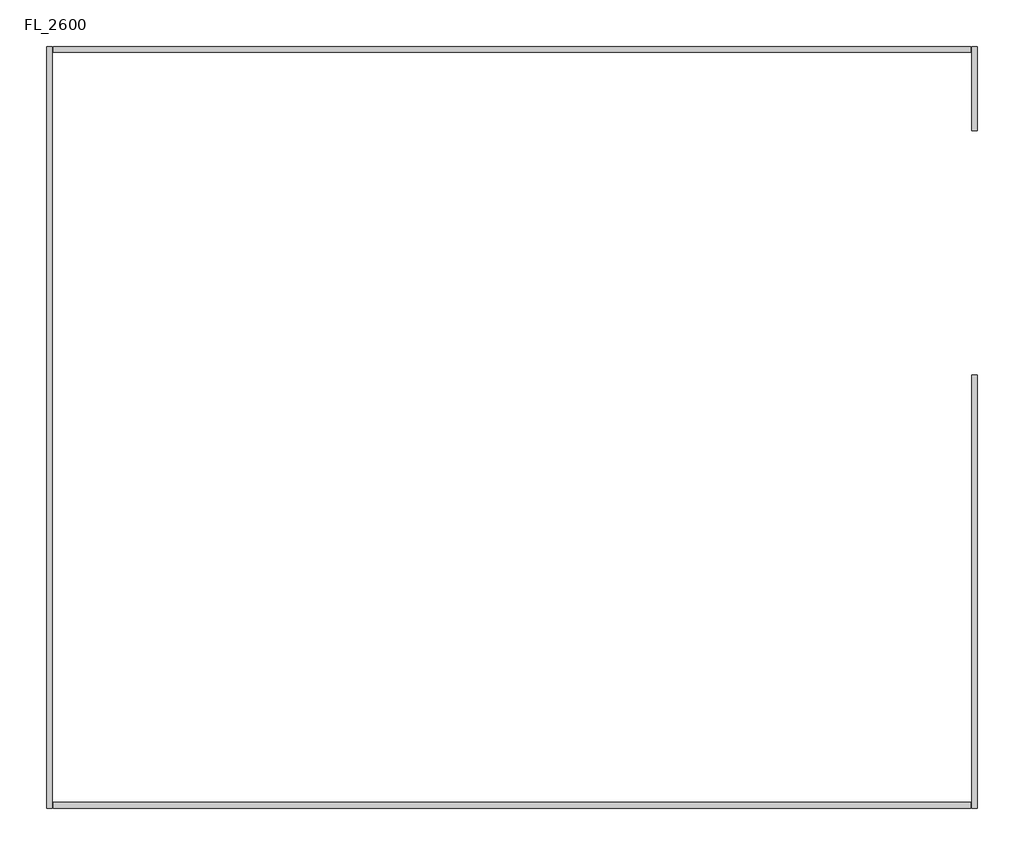
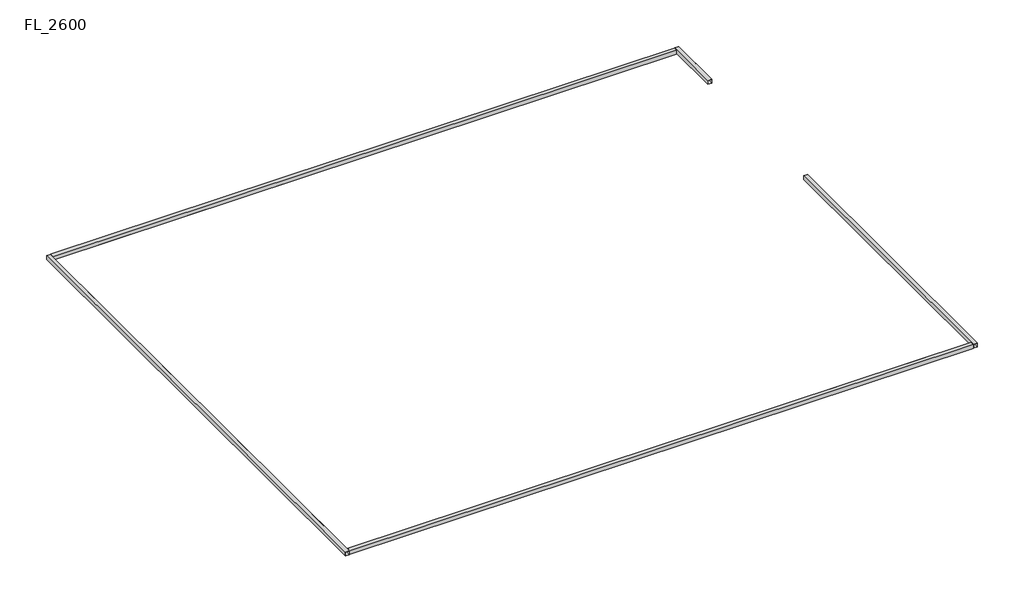
# One storey: 5 beams.
"""IFC4 building model written with IfcOpenShell, lengths in millimetres."""

import ifcopenshell
import ifcopenshell.guid

model = None  # the IFC model being written
_history = None  # IfcOwnerHistory: only IFC2X3 demands one
_inside = {}  # id of a spatial element -> (the spatial element, [elements in it])
_under = {}  # id of a project, library or spatial element -> (it, [spatial elements below it])
_declared = {}  # id of a project -> (the project, [libraries it declares])
_typed = {}  # id of a type object -> (the type object, [elements of that type])
_made_of = {}  # id of a material, layer set ... -> (it, [elements and type objects made of it])


def new_model(schema):
    """Start an empty IFC model of exactly this schema.

    Asked for "IFC4X3", IfcOpenShell would pick the latest addendum, in which some entities
    have other attributes; the version numbers below select the first issue.
    IFC2X3 requires an IfcOwnerHistory on every rooted entity: one is made here for all.
    """
    global model, _history
    if schema == "IFC4X3":
        model = ifcopenshell.file(schema_version=(4, 3, 0, 0))
    else:
        model = ifcopenshell.file(schema=schema)
    _inside.clear()
    _under.clear()
    _declared.clear()
    _typed.clear()
    _made_of.clear()
    _history = None
    if model.schema == "IFC2X3":
        org = make("IfcOrganization", Name="unknown")
        user = make(
            "IfcPersonAndOrganization",
            ThePerson=make("IfcPerson", FamilyName="unknown"),
            TheOrganization=org,
        )
        app = make(
            "IfcApplication",
            ApplicationDeveloper=org,
            Version="unknown",
            ApplicationFullName="unknown",
            ApplicationIdentifier="unknown",
        )
        _history = make(
            "IfcOwnerHistory",
            OwningUser=user,
            OwningApplication=app,
            ChangeAction="ADDED",
            CreationDate=0,
        )
    return model


def make(cls, **values):
    """One entity of the class cls with the attributes given. An attribute that is None is left unset."""
    return model.create_entity(
        cls, **{name: value for name, value in values.items() if value is not None}
    )


def rooted(cls, **values):
    """An entity with a GlobalId (a new one), such as an element, a storey or a relation."""
    return make(cls, GlobalId=ifcopenshell.guid.new(), OwnerHistory=_history, **values)


def si_unit(unit_type, name, prefix=None):
    """IfcSIUnit, for example si_unit("LENGTHUNIT", "METRE", prefix="MILLI")."""
    return make("IfcSIUnit", UnitType=unit_type, Prefix=prefix, Name=name)


def assignment(units):
    """IfcUnitAssignment: the units of a project."""
    return None if units is None else make("IfcUnitAssignment", Units=units)


def point(xyz):
    """IfcCartesianPoint."""
    return None if xyz is None else make("IfcCartesianPoint", Coordinates=xyz)


def direction(xyz):
    """IfcDirection."""
    return None if xyz is None else make("IfcDirection", DirectionRatios=xyz)


def frame(location, z_axis=None, x_axis=None):
    """IfcAxis2Placement3D, a coordinate frame: its origin and axes. An axis left out is left unset."""
    return make(
        "IfcAxis2Placement3D",
        Location=point(location),
        Axis=direction(z_axis),
        RefDirection=direction(x_axis),
    )


def origin():
    """The frame at (0, 0, 0) with its axes left unset."""
    return frame((0.0, 0.0, 0.0))


def place(relative_to, where):
    """IfcLocalPlacement: puts the frame where relative to a parent placement (None: the world)."""
    return make(
        "IfcLocalPlacement", PlacementRelTo=relative_to, RelativePlacement=where
    )


def context(
    kind, dimensions, precision=None, world=None, true_north=None, identifier=None
):
    """IfcGeometricRepresentationContext, for example the 3D "Model" context."""
    return make(
        "IfcGeometricRepresentationContext",
        ContextIdentifier=identifier,
        ContextType=kind,
        CoordinateSpaceDimension=dimensions,
        Precision=precision,
        WorldCoordinateSystem=world,
        TrueNorth=true_north,
    )


def project(units=None, contexts=None):
    """IfcProject with its units and contexts."""
    return rooted(
        "IfcProject",
        Name="project",
        RepresentationContexts=contexts,
        UnitsInContext=assignment(units),
    )


def spatial(cls, under=None, at=None, **own):
    """A site, building, storey or space (cls), placed at a placement, below another one or the project."""
    s = rooted(cls, ObjectPlacement=at, **own)
    if under is not None:
        _under.setdefault(under.id(), (under, []))[1].append(s)
    return s


def polyline(points):
    """IfcPolyline through the points."""
    return make("IfcPolyline", Points=[point(p) for p in points])


def outline(outer, holes=None, kind="AREA"):
    """IfcArbitraryClosedProfileDef: a profile drawn as a closed curve; with holes, ...WithVoids."""
    if holes is None:
        return make("IfcArbitraryClosedProfileDef", ProfileType=kind, OuterCurve=outer)
    return make(
        "IfcArbitraryProfileDefWithVoids",
        ProfileType=kind,
        OuterCurve=outer,
        InnerCurves=holes,
    )


def extrude(swept, where, along, depth):
    """IfcExtrudedAreaSolid: the profile swept, set in the frame where, extruded along a direction by depth."""
    return make(
        "IfcExtrudedAreaSolid",
        SweptArea=swept,
        Position=where,
        ExtrudedDirection=direction(along),
        Depth=depth,
    )


def shape(context_of_items, identifier, shape_type, items):
    """IfcShapeRepresentation: the items that make up one representation, for example the "Body"."""
    return make(
        "IfcShapeRepresentation",
        ContextOfItems=context_of_items,
        RepresentationIdentifier=identifier,
        RepresentationType=shape_type,
        Items=items,
    )


def source(mapping_origin, context_of_items, identifier, shape_type, items):
    """IfcRepresentationMap: a shape defined once, which mapped items show again and again."""
    return make(
        "IfcRepresentationMap",
        MappingOrigin=mapping_origin,
        MappedRepresentation=shape(context_of_items, identifier, shape_type, items),
    )


def transform(
    local_origin,
    x_axis=None,
    y_axis=None,
    z_axis=None,
    scale=None,
    scale2=None,
    scale3=None,
    uniform=True,
):
    """IfcCartesianTransformationOperator3D, or its non-uniform kind. x_axis, y_axis, z_axis: its Axis1, 2, 3."""
    if uniform:
        return make(
            "IfcCartesianTransformationOperator3D",
            Axis1=direction(x_axis),
            Axis2=direction(y_axis),
            LocalOrigin=point(local_origin),
            Scale=scale,
            Axis3=direction(z_axis),
        )
    return make(
        "IfcCartesianTransformationOperator3DnonUniform",
        Axis1=direction(x_axis),
        Axis2=direction(y_axis),
        LocalOrigin=point(local_origin),
        Scale=scale,
        Axis3=direction(z_axis),
        Scale2=scale2,
        Scale3=scale3,
    )


def mapped(mapping_source, mapping_target):
    """IfcMappedItem: shows the shape of a source again, moved by a transform."""
    return make(
        "IfcMappedItem", MappingSource=mapping_source, MappingTarget=mapping_target
    )


def made_of(thing, what):
    """Note that an element or type object is made of a material, layer set ...; save() writes the relation."""
    if what is not None:
        _made_of.setdefault(what.id(), (what, []))[1].append(thing)
    return thing


def element(
    cls,
    number,
    at=None,
    inside=None,
    cuts=None,
    type_object=None,
    material=None,
    context=None,
    identifier="Body",
    shape_type=None,
    held_by="IfcProductDefinitionShape",
    body=None,
    shapes=None,
    **own,
):
    """One element of the class cls, such as IfcWall. Its Tag is "e" and its number.

    at: its placement. inside: the storey or other place that contains it. cuts: it is an
    opening in that element (IfcRelVoidsElement). A single representation is given by context,
    identifier, shape_type and body (its items); several are given by shapes. held_by: the class
    of the entity that holds the representations. save() writes the other relations.
    """
    e = rooted(cls, Tag="e%d" % number, ObjectPlacement=at, **own)
    if body is not None:
        shapes = [shape(context, identifier, shape_type, body)]
    if shapes is not None:
        e.Representation = make(held_by, Representations=shapes)
    if inside is not None:
        _inside.setdefault(inside.id(), (inside, []))[1].append(e)
    if cuts is not None:
        rooted(
            "IfcRelVoidsElement", RelatingBuildingElement=cuts, RelatedOpeningElement=e
        )
    if type_object is not None:
        _typed.setdefault(type_object.id(), (type_object, []))[1].append(e)
    return made_of(e, material)


def aggregate(whole, parts):
    """IfcRelAggregates: a whole, such as a stair, and the parts it consists of."""
    return rooted("IfcRelAggregates", RelatingObject=whole, RelatedObjects=parts)


def save(model, path):
    """Write the relations noted so far, then the file.

    IfcRelAggregates (storeys below a building ...), IfcRelContainedInSpatialStructure (elements
    in a storey), IfcRelDefinesByType, IfcRelAssociatesMaterial and IfcRelDeclares: one each for
    every whole, place, type object, material and project.
    """
    for whole, parts in _under.values():
        aggregate(whole, parts)
    for where, things in _inside.values():
        rooted(
            "IfcRelContainedInSpatialStructure",
            RelatedElements=things,
            RelatingStructure=where,
        )
    for kind, things in _typed.values():
        rooted("IfcRelDefinesByType", RelatedObjects=things, RelatingType=kind)
    for what, things in _made_of.values():
        rooted("IfcRelAssociatesMaterial", RelatedObjects=things, RelatingMaterial=what)
    for by, libraries in _declared.values():
        rooted("IfcRelDeclares", RelatingContext=by, RelatedDefinitions=libraries)
    model.write(path)


def steel_rectangular_beam_bm125_rt_100x100x4_0_fd47acba(model_context):
    return source(origin(), model_context, "Body", "SweptSolid", [
        extrude(outline(polyline([(-50.0, 50.0), (50.0, 50.0), (50.0, -50.0), (-50.0, -50.0), (-50.0, 50.0)]), holes=[polyline([(46.0, -46.0), (46.0, 46.0), (-46.0, 46.0), (-46.0, -46.0), (46.0, -46.0)])]), frame((-7887.3, 0.0, 0.0), z_axis=(1.0, 0.0, 0.0), x_axis=(0.0, 1.0, 0.0)), (0.0, 0.0, 1.0), 15774.6),
        extrude(outline(polyline([(-50.0, 50.0), (50.0, 50.0), (50.0, -50.0), (-50.0, -50.0), (-50.0, 50.0)]), holes=[polyline([(46.0, -46.0), (46.0, 46.0), (-46.0, 46.0), (-46.0, -46.0), (46.0, -46.0)])]), frame((-7887.3, 0.0, 0.0), z_axis=(1.0, 0.0, 0.0), x_axis=(0.0, 1.0, 0.0)), (0.0, 0.0, 1.0), 15774.6),
        extrude(outline(polyline([(-50.0, 50.0), (50.0, 50.0), (50.0, -50.0), (-50.0, -50.0), (-50.0, 50.0)]), holes=[polyline([(46.0, -46.0), (46.0, 46.0), (-46.0, 46.0), (-46.0, -46.0), (46.0, -46.0)])]), frame((-7887.3, 0.0, 0.0), z_axis=(1.0, 0.0, 0.0), x_axis=(0.0, 1.0, 0.0)), (0.0, 0.0, 1.0), 15774.6),
        extrude(outline(polyline([(-50.0, 50.0), (50.0, 50.0), (50.0, -50.0), (-50.0, -50.0), (-50.0, 50.0)]), holes=[polyline([(46.0, -46.0), (46.0, 46.0), (-46.0, 46.0), (-46.0, -46.0), (46.0, -46.0)])]), frame((-7887.3, 0.0, 0.0), z_axis=(1.0, 0.0, 0.0), x_axis=(0.0, 1.0, 0.0)), (0.0, 0.0, 1.0), 15774.6),
    ])


def steel_rectangular_beam_bm125_rt_100x100x4_0_2c93a6f0(model_context):
    return source(origin(), model_context, "Body", "SweptSolid", [
        extrude(outline(polyline([(-50.0, 50.0), (50.0, 50.0), (50.0, -50.0), (-50.0, -50.0), (-50.0, 50.0)]), holes=[polyline([(46.0, -46.0), (46.0, 46.0), (-46.0, 46.0), (-46.0, -46.0), (46.0, -46.0)])]), frame((-6550.0, 0.0, 0.0), z_axis=(1.0, 0.0, 0.0), x_axis=(0.0, 1.0, 0.0)), (0.0, 0.0, 1.0), 13100.0),
        extrude(outline(polyline([(-50.0, 50.0), (50.0, 50.0), (50.0, -50.0), (-50.0, -50.0), (-50.0, 50.0)]), holes=[polyline([(46.0, -46.0), (46.0, 46.0), (-46.0, 46.0), (-46.0, -46.0), (46.0, -46.0)])]), frame((-6550.0, 0.0, 0.0), z_axis=(1.0, 0.0, 0.0), x_axis=(0.0, 1.0, 0.0)), (0.0, 0.0, 1.0), 13100.0),
        extrude(outline(polyline([(-50.0, 50.0), (50.0, 50.0), (50.0, -50.0), (-50.0, -50.0), (-50.0, 50.0)]), holes=[polyline([(46.0, -46.0), (46.0, 46.0), (-46.0, 46.0), (-46.0, -46.0), (46.0, -46.0)])]), frame((-6550.0, 0.0, 0.0), z_axis=(1.0, 0.0, 0.0), x_axis=(0.0, 1.0, 0.0)), (0.0, 0.0, 1.0), 13100.0),
        extrude(outline(polyline([(-50.0, 50.0), (50.0, 50.0), (50.0, -50.0), (-50.0, -50.0), (-50.0, 50.0)]), holes=[polyline([(46.0, -46.0), (46.0, 46.0), (-46.0, 46.0), (-46.0, -46.0), (46.0, -46.0)])]), frame((-6550.0, 0.0, 0.0), z_axis=(1.0, 0.0, 0.0), x_axis=(0.0, 1.0, 0.0)), (0.0, 0.0, 1.0), 13100.0),
    ])


def steel_rectangular_beam_bm125_rt_100x100x4_0_60a5dd41(model_context):
    return source(origin(), model_context, "Body", "SweptSolid", [
        extrude(outline(polyline([(-50.0, 50.0), (50.0, 50.0), (50.0, -50.0), (-50.0, -50.0), (-50.0, 50.0)]), holes=[polyline([(46.0, -46.0), (46.0, 46.0), (-46.0, 46.0), (-46.0, -46.0), (46.0, -46.0)])]), frame((-3725.0, 0.0, 0.0), z_axis=(1.0, 0.0, 0.0), x_axis=(0.0, 1.0, 0.0)), (0.0, 0.0, 1.0), 7450.0),
        extrude(outline(polyline([(-50.0, 50.0), (50.0, 50.0), (50.0, -50.0), (-50.0, -50.0), (-50.0, 50.0)]), holes=[polyline([(46.0, -46.0), (46.0, 46.0), (-46.0, 46.0), (-46.0, -46.0), (46.0, -46.0)])]), frame((-3725.0, 0.0, 0.0), z_axis=(1.0, 0.0, 0.0), x_axis=(0.0, 1.0, 0.0)), (0.0, 0.0, 1.0), 7450.0),
        extrude(outline(polyline([(-50.0, 50.0), (50.0, 50.0), (50.0, -50.0), (-50.0, -50.0), (-50.0, 50.0)]), holes=[polyline([(46.0, -46.0), (46.0, 46.0), (-46.0, 46.0), (-46.0, -46.0), (46.0, -46.0)])]), frame((-3725.0, 0.0, 0.0), z_axis=(1.0, 0.0, 0.0), x_axis=(0.0, 1.0, 0.0)), (0.0, 0.0, 1.0), 7450.0),
        extrude(outline(polyline([(-50.0, 50.0), (50.0, 50.0), (50.0, -50.0), (-50.0, -50.0), (-50.0, 50.0)]), holes=[polyline([(46.0, -46.0), (46.0, 46.0), (-46.0, 46.0), (-46.0, -46.0), (46.0, -46.0)])]), frame((-3725.0, 0.0, 0.0), z_axis=(1.0, 0.0, 0.0), x_axis=(0.0, 1.0, 0.0)), (0.0, 0.0, 1.0), 7450.0),
    ])


def steel_rectangular_beam_bm125_rt_100x100x4_0_366960fc(model_context):
    return source(origin(), model_context, "Body", "SweptSolid", [
        extrude(outline(polyline([(-50.0, 50.0), (50.0, 50.0), (50.0, -50.0), (-50.0, -50.0), (-50.0, 50.0)]), holes=[polyline([(46.0, -46.0), (46.0, 46.0), (-46.0, 46.0), (-46.0, -46.0), (46.0, -46.0)])]), frame((-725.0, 0.0, 0.0), z_axis=(1.0, 0.0, 0.0), x_axis=(0.0, 1.0, 0.0)), (0.0, 0.0, 1.0), 1450.0),
        extrude(outline(polyline([(-50.0, 50.0), (50.0, 50.0), (50.0, -50.0), (-50.0, -50.0), (-50.0, 50.0)]), holes=[polyline([(46.0, -46.0), (46.0, 46.0), (-46.0, 46.0), (-46.0, -46.0), (46.0, -46.0)])]), frame((-725.0, 0.0, 0.0), z_axis=(1.0, 0.0, 0.0), x_axis=(0.0, 1.0, 0.0)), (0.0, 0.0, 1.0), 1450.0),
        extrude(outline(polyline([(-50.0, 50.0), (50.0, 50.0), (50.0, -50.0), (-50.0, -50.0), (-50.0, 50.0)]), holes=[polyline([(46.0, -46.0), (46.0, 46.0), (-46.0, 46.0), (-46.0, -46.0), (46.0, -46.0)])]), frame((-725.0, 0.0, 0.0), z_axis=(1.0, 0.0, 0.0), x_axis=(0.0, 1.0, 0.0)), (0.0, 0.0, 1.0), 1450.0),
        extrude(outline(polyline([(-50.0, 50.0), (50.0, 50.0), (50.0, -50.0), (-50.0, -50.0), (-50.0, 50.0)]), holes=[polyline([(46.0, -46.0), (46.0, 46.0), (-46.0, 46.0), (-46.0, -46.0), (46.0, -46.0)])]), frame((-725.0, 0.0, 0.0), z_axis=(1.0, 0.0, 0.0), x_axis=(0.0, 1.0, 0.0)), (0.0, 0.0, 1.0), 1450.0),
    ])


model = new_model("IFC4")

# Units and contexts
model_context = context("Model", 3, world=origin())
ifc_project = project(units=[si_unit("LENGTHUNIT", "METRE", prefix="MILLI")], contexts=[model_context])

# Site, building, storey
site = spatial("IfcSite", under=ifc_project)
building = spatial("IfcBuilding", under=site)
storey = spatial("IfcBuildingStorey", under=building, Name="FL_2600", Elevation=2600.0)

# Beams
placement = place(None, origin())
steel_rectangular_beam_bm125_rt_100x100x4_0_shape = steel_rectangular_beam_bm125_rt_100x100x4_0_fd47acba(model_context)
element("IfcBeam", 1, ObjectType="Steel-Rectangular-Beam : BM125_RT-100x100x4.0", at=placement, inside=storey, context=model_context, shape_type="MappedRepresentation", body=[
    mapped(steel_rectangular_beam_bm125_rt_100x100x4_0_shape, transform((6100.0, 10094.5382614, 2550.0), x_axis=(1.0, 0.0, 0.0), y_axis=(0.0, 1.0, 0.0), z_axis=(0.0, 0.0, 1.0))),
])
element("IfcBeam", 2, ObjectType="Steel-Rectangular-Beam : BM125_RT-100x100x4.0", at=placement, inside=storey, context=model_context, shape_type="MappedRepresentation", body=[
    mapped(steel_rectangular_beam_bm125_rt_100x100x4_0_shape, transform((6100.0, 23094.5382614, 2550.0), x_axis=(-1.0, 0.0, 0.0), y_axis=(0.0, -1.0, 0.0), z_axis=(0.0, 0.0, 1.0))),
])
steel_rectangular_beam_bm125_rt_100x100x4_0_2_shape = steel_rectangular_beam_bm125_rt_100x100x4_0_2c93a6f0(model_context)
element("IfcBeam", 3, ObjectType="Steel-Rectangular-Beam : BM125_RT-100x100x4.0", at=placement, inside=storey, context=model_context, shape_type="MappedRepresentation", body=[
    mapped(steel_rectangular_beam_bm125_rt_100x100x4_0_2_shape, transform((-1850.0, 16594.5382614, 2550.0), x_axis=(0.0, -1.0, 0.0), y_axis=(1.0, 0.0, 0.0), z_axis=(0.0, 0.0, 1.0))),
])
steel_rectangular_beam_bm125_rt_100x100x4_0_3_shape = steel_rectangular_beam_bm125_rt_100x100x4_0_60a5dd41(model_context)
element("IfcBeam", 4, ObjectType="Steel-Rectangular-Beam : BM125_RT-100x100x4.0", at=placement, inside=storey, context=model_context, shape_type="MappedRepresentation", body=[
    mapped(steel_rectangular_beam_bm125_rt_100x100x4_0_3_shape, transform((14050.0, 13769.5382614, 2550.0), x_axis=(0.0, 1.0, 0.0), y_axis=(-1.0, 0.0, 0.0), z_axis=(0.0, 0.0, 1.0))),
])
steel_rectangular_beam_bm125_rt_100x100x4_0_4_shape = steel_rectangular_beam_bm125_rt_100x100x4_0_366960fc(model_context)
element("IfcBeam", 5, ObjectType="Steel-Rectangular-Beam : BM125_RT-100x100x4.0", at=placement, inside=storey, context=model_context, shape_type="MappedRepresentation", body=[
    mapped(steel_rectangular_beam_bm125_rt_100x100x4_0_4_shape, transform((14050.0, 22419.5382614, 2550.0), x_axis=(0.0, 1.0, 0.0), y_axis=(-1.0, 0.0, 0.0), z_axis=(0.0, 0.0, 1.0))),
])

save(model, "model.ifc")

# Revit data of these elements
# Project information
#   Project ISM Data = "<?xml version=\"1.0\" encoding=\"utf-16\"?><ism schema_version=\"03.00\"><section_positioning><element family_name=\"CO_RC_REC\" symbol_name=\"CCC12_Rec_450x450\" section_id=\"F2ADF140-E21A-4820-8170-6F63D956DCAD\" category=\"OST_StructuralColumns\" mirror_y=\"0\" mirror_x=\"0\" /><element family_name=\"CO_RC_REC\" symbol_name=\"CCC12_Rec_450x450\" section_id=\"B35A310E-4F33-462b-819C-3ADD300C0CEB\" category=\"OST_StructuralColumns\" mirror_y=\"0\" mirror_x=\"0\" /><element family_name=\"CO_RC_REC\" symbol_name=\"CCC12_Rec_450x450\" section_id=\"711054EC-0DB2-46e3-AD20-004560300C00\" category=\"OST_StructuralColumns\" mirror_y=\"0\" mirror_x=\"0\" /><element family_name=\"CO_RC_REC\" symbol_name=\"300 x 450\" section_id=\"B5C54EC9-8EBD-4860-AB72-EF5791AED394\" category=\"OST_StructuralColumns\" mirror_y=\"0\" mirror_x=\"0\" /><element family_name=\"GI_RC_C\" symbol_name=\"SGC11_400x500\" section_id=\"0A7B8D02-9EA4-4aa9-A41A-E30BB5B6B6C5\" category=\"OST_StructuralFraming\" mirror_y=\"0\" mirror_x=\"0\" /><element family_name=\"GI_RC_C\" symbol_name=\"SGC11_400x500\" section_id=\"714BBD27-DB58-47da-B54C-5806291C2D3C\" category=\"OST_StructuralFraming\" mirror_y=\"0\" mirror_x=\"0\" /><element family_name=\"GI_RC_C\" symbol_name=\"SGC11_400x500\" section_id=\"F36E62C1-13EE-4807-A3C1-899E23E0BEDE\" category=\"OST_StructuralFraming\" mirror_y=\"0\" mirror_x=\"0\" /><element family_name=\"GI_RC_C\" symbol_name=\"SGC11_400x500\" section_id=\"F5448801-679E-44d6-8F46-E676344F8165\" category=\"OST_StructuralFraming\" mirror_y=\"0\" mirror_x=\"0\" /><element family_name=\"GI_RC_C\" symbol_name=\"SGC11_400x600\" section_id=\"05D74241-6318-4cac-95F5-7B878260D5B5\" category=\"OST_StructuralFraming\" mirror_y=\"0\" mirror_x=\"0\" /><element family_name=\"GI_RC_C\" symbol_name=\"SGC11_400x500\" section_id=\"846DCB0C-E06B-4978-9D43-E1CC0FDE7595\" category=\"OST_StructuralFraming\" mirror_y=\"0\" mirror_x=\"0\" /><element family_name=\"GI_RC_C\" symbol_name=\"SGC11_400x500\" section_id=\"2ADF82B8-986D-4f44-85DE-89D921292160\" category=\"OST_StructuralFraming\" mirror_y=\"0\" mirror_x=\"0\" /><element family_name=\"GI_RC_C\" symbol_name=\"SGC11_400x500\" section_id=\"7AF371ED-051B-4a30-8826-11F11C212B73\" category=\"OST_StructuralFraming\" mirror_y=\"0\" mirror_x=\"0\" /><element family_name=\"GI_RC_C\" symbol_name=\"SGC11_400x500\" section_id=\"2FE74006-ADDA-412f-A522-853919E62B4D\" category=\"OST_StructuralFraming\" mirror_y=\"0\" mirror_x=\"0\" /><element family_name=\"GI_RC_C\" symbol_name=\"SGC11_400x500\" section_id=\"09B63641-D581-4a6c-A18E-54C17EC989A4\" category=\"OST_StructuralFraming\" mirror_y=\"0\" mirror_x=\"0\" /><element family_name=\"GI_RC_C\" symbol_name=\"SGC11_400x500\" section_id=\"0DD6B52A-77D0-45a1-82B1-8236ED57078C\" category=\"OST_StructuralFraming\" mirror_y=\"0\" mirror_x=\"0\" /><element family_name=\"GI_RC_C\" symbol_name=\"SGC11_400x500\" section_id=\"35D311D2-DEB8-4469-97DE-110B6DF5B84D\" category=\"OST_StructuralFraming\" mirror_y=\"0\" mirror_x=\"0\" /><element family_name=\"GI_RC_C\" symbol_name=\"SGC11_400x500\" section_id=\"0D3CCDE5-CFF9-431b-A4BD-01BF6636D6BD\" category=\"OST_StructuralFraming\" mirror_y=\"0\" mirror_x=\"0\" /><element family_name=\"GI_RC_C\" symbol_name=\"SGC11_400x500\" section_id=\"C62B2A5B-024A-47ac-B030-C17A67E64A7B\" category=\"OST_StructuralFraming\" mirror_y=\"0\" mirror_x=\"0\" /><element family_name=\"GI_RC_C\" symbol_name=\"SGC11_400x500\" section_id=\"944C6E43-E607-48c3-8358-9E6CB88346E7\" category=\"OST_StructuralFraming\" mirror_y=\"0\" mirror_x=\"0\" /><element family_name=\"GI_RC_C\" symbol_name=\"SGC11_400x500\" section_id=\"A4B1F42D-B1C2-4ad2-8AD6-DB0D5E05998D\" category=\"OST_StructuralFraming\" mirror_y=\"0\" mirror_x=\"0\" /><element family_name=\"GI_RC_C\" symbol_name=\"SGC11_400x500\" section_id=\"007E6C70-1139-4b48-B003-C76FAD4C249A\" category=\"OST_StructuralFraming\" mirror_y=\"0\" mirror_x=\"0\" /><element family_name=\"GI_RC_C\" symbol_name=\"SGC11_400x500\" section_id=\"9941AC94-F03A-464c-9912-04590E0C31E0\" category=\"OST_StructuralFraming\" mirror_y=\"0\" mirror_x=\"0\" /><element family_name=\"GI_RC_C\" symbol_name=\"SGC11_400x500\" section_id=\"CFD98B8D-8FF4-4e71-A909-0FE7DBCE924E\" category=\"OST_StructuralFraming\" mirror_y=\"0\" mirror_x=\"0\" /><element family_name=\"GI_RC_C\" symbol_name=\"SGC11_400x500\" section_id=\"58262161-98E6-45c8-B2BD-4508105FF662\" category=\"OST_StructuralFraming\" mirror_y=\"0\" mirror_x=\"0\" /><element family_name=\"GI_RC_C\" symbol_name=\"SGC11_400x500\" section_id=\"66AB4841-610A-4883-97F7-1282A56484E1\" category=\"OST_StructuralFraming\" mirror_y=\"0\" mirror_x=\"0\" /><element family_name=\"GI_RC_C\" symbol_name=\"SGC11_400x500\" section_id=\"D2B324BE-BBD6-49da-9730-60EA7AD4D3A0\" category=\"OST_StructuralFraming\" mirror_y=\"0\" mirror_x=\"0\" /><element family_name=\"GI_RC_C\" symbol_name=\"SGC11_400x500\" section_id=\"92A8ECE7-C053-46b1-92ED-F2C041617E7B\" category=\"OST_StructuralFraming\" mirror_y=\"0\" mirror_x=\"0\" /><element family_name=\"GI_RC_C\" symbol_name=\"SGC11_400x500\" section_id=\"B4C4BDB0-65C4-4016-9C78-DBD77E229523\" category=\"OST_StructuralFraming\" mirror_y=\"0\" mirror_x=\"0\" /><element family_name=\"GI_RC_C\" symbol_name=\"SGC11_400x500\" section_id=\"57270646-162F-4c83-BDB7-A5FBEA9120BD\" category=\"OST_StructuralFraming\" mirror_y=\"0\" mirror_x=\"0\" /><element family_name=\"GI_RC_C\" symbol_name=\"SGC11_400x500\" section_id=\"BDEF733F-00AA-4eee-B6C6-50229FC1D236\" category=\"OST_StructuralFraming\" mirror_y=\"0\" mirror_x=\"0\" /><element family_name=\"GI_RC_C\" symbol_name=\"SGC11_400x500\" section_id=\"84A94E1E-3074-40f4-9690-97191755F019\" category=\"OST_StructuralFraming\" mirror_y=\"0\" mirror_x=\"0\" /><element family_name=\"GI_RC_C\" symbol_name=\"SGC11_400x500\" section_id=\"8A7D913D-7967-4718-912D-B83DF0AD2EDD\" category=\"OST_StructuralFraming\" mirror_y=\"0\" mirror_x=\"0\" /><element family_name=\"GI_RC_C\" symbol_name=\"SGC11_400x500\" section_id=\"83553D70-90FA-469c-B5C3-EF03F3FC6475\" category=\"OST_StructuralFraming\" mirror_y=\"0\" mirror_x=\"0\" /><element family_name=\"GI_RC_C\" symbol_name=\"SGC11_400x500\" section_id=\"6880C1E4-C50B-4c1b-B61C-23F2D8C46873\" category=\"OST_StructuralFraming\" mirror_y=\"0\" mirror_x=\"0\" /><element family_name=\"GI_RC_C\" symbol_name=\"SGC11_400x500\" section_id=\"08594C43-CD40-47de-A3BA-8BFB47F64994\" category=\"OST_StructuralFraming\" mirror_y=\"0\" mirror_x=\"0\" /><element family_name=\"GI_RC_C\" symbol_name=\"SGC11_400x500\" section_id=\"7D2E11FA-A5E1-4434-B9BE-AABA1A16CA03\" category=\"OST_StructuralFraming\" mirror_y=\"0\" mirror_x=\"0\" /><element family_name=\"GI_RC_C\" symbol_name=\"SGC11_400x500\" section_id=\"D892DFA4-5441-4ad2-A390-253492293B1B\" category=\"OST_StructuralFraming\" mirror_y=\"0\" mirror_x=\"0\" /><element family_name=\"GI_RC_C\" symbol_name=\"SGC11_400x500\" section_id=\"E5A32FE6-89C4-49f1-B3B9-1CABE7C48A4D\" category=\"OST_StructuralFraming\" mirror_y=\"0\" mirror_x=\"0\" /><element family_name=\"GI_RC_C\" symbol_name=\"SGC11_400x500\" section_id=\"8AE872C2-5DBE-47c5-934B-7E964A84B589\" category=\"OST_StructuralFraming\" mirror_y=\"0\" mirror_x=\"0\" /><element family_name=\"GI_RC_C\" symbol_name=\"SGC11_400x500\" section_id=\"3C847B60-488A-4604-A400-16A3A65E919B\" category=\"OST_StructuralFraming\" mirror_y=\"0\" mirror_x=\"0\" /><element family_name=\"GI_RC_C\" symbol_name=\"SGC11_400x500\" section_id=\"DBEC432A-3F7B-4266-AD99-2A937DC70BCF\" category=\"OST_StructuralFraming\" mirror_y=\"0\" mirror_x=\"0\" /><element family_name=\"GI_RC_C\" symbol_name=\"SGC11_400x500\" section_id=\"59403DD6-7A51-48aa-A3BE-962457E6F10E\" category=\"OST_StructuralFraming\" mirror_y=\"0\" mirror_x=\"0\" /><element family_name=\"GI_RC_C\" symbol_name=\"SGC11_400x500\" section_id=\"11CDDF5D-38B6-43b2-A291-FC188BE232BC\" category=\"OST_StructuralFraming\" mirror_y=\"0\" mirror_x=\"0\" /><element family_name=\"GI_RC_C\" symbol_name=\"SGC11_400x500\" section_id=\"10BF2843-EFC9-4136-933C-5B270D970277\" category=\"OST_StructuralFraming\" mirror_y=\"0\" mirror_x=\"0\" /><element family_name=\"GI_RC_C\" symbol_name=\"SGC11_400x500\" section_id=\"E1B09A9C-F6C6-47d9-976B-E313C0E3F52B\" category=\"OST_StructuralFraming\" mirror_y=\"0\" mirror_x=\"0\" /><element family_name=\"GI_RC_C\" symbol_name=\"SGC11_400x500\" section_id=\"A3A22EC3-26C8-4588-A0AB-AFAE02DF267E\" category=\"OST_StructuralFraming\" mirror_y=\"0\" mirror_x=\"0\" /><element family_name=\"GI_RC_C\" symbol_name=\"SGC11_400x500\" section_id=\"114828FC-BDC1-4343-9119-BCB5395DAA64\" category=\"OST_StructuralFraming\" mirror_y=\"0\" mirror_x=\"0\" /><element family_name=\"GI_RC_C\" symbol_name=\"SGC11_400x500\" section_id=\"797626F9-3558-4623-826F-15FB93088CB3\" category=\"OST_StructuralFraming\" mirror_y=\"0\" mirror_x=\"0\" /><element family_name=\"GI_RC_C\" symbol_name=\"SGC11_400x500\" section_id=\"4BF369CD-DF09-4346-96CB-C6C6380A2599\" category=\"OST_StructuralFraming\" mirror_y=\"0\" mirror_x=\"0\" /><element family_name=\"GI_RC_C\" symbol_name=\"SGC11_400x500\" section_id=\"722B46BA-61C4-44a1-9ECF-325B60B6688D\" category=\"OST_StructuralFraming\" mirror_y=\"0\" mirror_x=\"0\" /><element family_name=\"GI_RC_C\" symbol_name=\"SGC11_400x500\" section_id=\"C33DBE84-19C1-4379-AB6E-A41F7420F18C\" category=\"OST_StructuralFraming\" mirror_y=\"0\" mirror_x=\"0\" /><element family_name=\"GI_RC_C\" symbol_name=\"SGC11_400x500\" section_id=\"1F2D3B75-66F2-4d88-A1DD-647969477B86\" category=\"OST_StructuralFraming\" mirror_y=\"0\" mirror_x=\"0\" /><element family_name=\"GI_RC_C\" symbol_name=\"SGC11_400x500\" section_id=\"DFBF96B2-410A-4f39-80C4-D8CF78561C93\" category=\"OST_StructuralFraming\" mirror_y=\"0\" mirror_x=\"0\" /><element family_name=\"GI_RC_C\" symbol_name=\"SGC11_400x500\" section_id=\"D6793CD3-AB64-417c-9C28-8B18A0A2D336\" category=\"OST_StructuralFraming\" mirror_y=\"0\" mirror_x=\"0\" /><element family_name=\"GI_RC_C\" symbol_name=\"SGC11_400x500\" section_id=\"90884AC0-EA00-4caa-86E1-E6B886FD90ED\" category=\"OST_StructuralFraming\" mirror_y=\"0\" mirror_x=\"0\" /><element family_name=\"GI_RC_C\" symbol_name=\"SGC11_400x500\" section_id=\"64BC7B89-F7C8-4dae-A5C8-F10DF9E5F6BA\" category=\"OST_StructuralFraming\" mirror_y=\"0\" mirror_x=\"0\" /><element family_name=\"GI_RC_C\" symbol_name=\"SGC11_400x500\" section_id=\"D82E4D85-2728-40e5-9F60-1C7FB2990D78\" category=\"OST_StructuralFraming\" mirror_y=\"0\" mirror_x=\"0\" /><element family_name=\"GI_RC_C\" symbol_name=\"SGC11_400x500\" section_id=\"1E6D05B9-BF84-4669-AA27-948ADA1D511E\" category=\"OST_StructuralFraming\" mirror_y=\"0\" mirror_x=\"0\" /><element family_name=\"GI_RC_C\" symbol_name=\"SGC11_400x500\" section_id=\"73608CB2-EB94-466e-883D-814030EF49D6\" category=\"OST_StructuralFraming\" mirror_y=\"0\" mirror_x=\"0\" /><element family_name=\"GI_RC_C\" symbol_name=\"SGC11_400x500\" section_id=\"4EAF07EF-4E08-4065-9F08-BF69D4413867\" category=\"OST_StructuralFraming\" mirror_y=\"1\" mirror_x=\"1\" /></section_positioning><surface_member_mappings /><element_binding><element revit_id=\"0aa8b22b-49cd-4eb2-b994-d423f7aad482-0014435e\" ism_id=\"637A3C89-B4B9-4EE4-9E04-FF73E7A5771D\" /><element revit_id=\"af7cfdda-f71a-4a09-bb03-63e0c16d5d93-00152efa\" ism_id=\"088C1743-AFAE-4D55-B14F-2330F3A79060\" /><element revit_id=\"af7cfdda-f71a-4a09-bb03-63e0c16d5d93-00152efc\" ism_id=\"38278b30-864a-4bde-bfee-6c2d4309b281\" /><element revit_id=\"af7cfdda-f71a-4a09-bb03-63e0c16d5d93-00152eff\" ism_id=\"e2895b00-887b-4cf1-92a9-c4855f67b579\" /><element revit_id=\"af7cfdda-f71a-4a09-bb03-63e0c16d5d93-00152f02\" ism_id=\"a6b13b86-1938-47ee-8937-754844bb71d9\" /><element revit_id=\"af7cfdda-f71a-4a09-bb03-63e0c16d5d93-00152f05\" ism_id=\"b3cdb4ae-01be-49a8-8521-dfb37fcb7a09\" /><element revit_id=\"af7cfdda-f71a-4a09-bb03-63e0c16d5d93-00152f08\" ism_id=\"0a200294-2d0f-43b2-a10b-c345be42008c\" /><element revit_id=\"af7cfdda-f71a-4a09-bb03-63e0c16d5d
#     93-00152f0a\" ism_id=\"434ac00d-0b75-408a-b526-bf8655b26baf\" /><element revit_id=\"af7cfdda-f71a-4a09-bb03-63e0c16d5d93-00152f0c\" ism_id=\"5e4f7e2a-2154-47cc-93bc-24e7bd197632\" /><element revit_id=\"af7cfdda-f71a-4a09-bb03-63e0c16d5d93-00152f0e\" ism_id=\"f1998cd9-044c-4f7a-99e6-248bc5b45dba\" /><element revit_id=\"af7cfdda-f71a-4a09-bb03-63e0c16d5d93-00152f10\" ism_id=\"6ca0e144-6dd7-4824-b6a4-c3599ffcc64c\" /><element revit_id=\"af7cfdda-f71a-4a09-bb03-63e0c16d5d93-00152f12\" ism_id=\"173f1f07-ca52-4750-b7f6-1ef0180c36ba\" /><element revit_id=\"af7cfdda-f71a-4a09-bb03-63e0c16d5d93-00152f15\" ism_id=\"29a619d1-86ac-46c7-a220-2e78769b313e\" /><element revit_id=\"af7cfdda-f71a-4a09-bb03-63e0c16d5d93-00152f17\" ism_id=\"de21b25d-6b5e-4da6-89ee-8b671f1287ec\" /><element revit_id=\"af7cfdda-f71a-4a09-bb03-63e0c16d5d93-00152f19\" ism_id=\"70cdf538-eeaa-48c4-9315-181e56578638\" /><element revit_id=\"af7cfdda-f71a-4a09-bb03-63e0c16d5d93-00152f1b\" ism_id=\"49734cf8-a963-4163-b104-a25bff74fff0\" /><element revit_id=\"af7cfdda-f71a-4a09-bb03-63e0c16d5d93-00152f1d\" ism_id=\"a5a98e28-e98d-4759-bcab-d40632bfc19f\" /><element revit_id=\"af7cfdda-f71a-4a09-bb03-63e0c16d5d93-00152f1f\" ism_id=\"ab6af08f-90da-4d2f-a66a-db65621b8e94\" /><element revit_id=\"af7cfdda-f71a-4a09-bb03-63e0c16d5d93-00152f21\" ism_id=\"a65b64ab-134d-4223-82b7-5e66d90bc276\" /><element revit_id=\"af7cfdda-f71a-4a09-bb03-63e0c16d5d93-00152f23\" ism_id=\"6a1f317f-8940-4af8-9522-8e6c47c0c3a6\" /><element revit_id=\"af7cfdda-f71a-4a09-bb03-63e0c16d5d93-00152f25\" ism_id=\"880c6aab-7058-4382-9d83-6c759bdcf822\" /><element revit_id=\"af7cfdda-f71a-4a09-bb03-63e0c16d5d93-00152f27\" ism_id=\"555977b1-6494-4ee8-b235-8bae97762787\" /><element revit_id=\"af7cfdda-f71a-4a09-bb03-63e0c16d5d93-00152f29\" ism_id=\"66c9b467-8c65-4f1e-9542-95b43d793e9b\" /><element revit_id=\"af7cfdda-f71a-4a09-bb03-63e0c16d5d93-00152f2b\" ism_id=\"217a9ce2-64ab-4115-836e-06014fa1b21e\" /><element revit_id=\"af7cfdda-f71a-4a09-bb03-63e0c16d5d93-00152f2d\" ism_id=\"f7fc30da-832d-44e7-bab3-dd115d25639e\" /><element revit_id=\"af7cfdda-f71a-4a09-bb03-63e0c16d5d93-00152f2f\" ism_id=\"715eb46c-1b8d-4226-a7c6-6c6c165bf34d\" /><element revit_id=\"af7cfdda-f71a-4a09-bb03-63e0c16d5d93-00152f31\" ism_id=\"ef53c2b2-6fcf-42d2-96ea-f30a899bf64f\" /><element revit_id=\"af7cfdda-f71a-4a09-bb03-63e0c16d5d93-00152f34\" ism_id=\"1aefa093-18ee-4a97-8178-1b1fb4b7aceb\" /><element revit_id=\"af7cfdda-f71a-4a09-bb03-63e0c16d5d93-00152f38\" ism_id=\"262f02a9-64ca-487b-befd-4b58d44dffa7\" /><element revit_id=\"af7cfdda-f71a-4a09-bb03-63e0c16d5d93-00152f3b\" ism_id=\"6f2442a8-c4c0-4b53-9d7f-7059d6ededd2\" /><element revit_id=\"af7cfdda-f71a-4a09-bb03-63e0c16d5d93-00152f3e\" ism_id=\"dd838df4-69c7-406c-93e1-418c01f5734f\" /><element revit_id=\"af7cfdda-f71a-4a09-bb03-63e0c16d5d93-00152f40\" ism_id=\"9dec5077-28a7-4c32-95d2-08813de6a916\" /><element revit_id=\"af7cfdda-f71a-4a09-bb03-63e0c16d5d93-00152f42\" ism_id=\"9370ae5f-9277-4bb3-917b-cb3f318800a8\" /><element revit_id=\"af7cfdda-f71a-4a09-bb03-63e0c16d5d93-00152f44\" ism_id=\"0f3f2c81-58b4-4698-b1be-75061a4a2ae1\" /><element revit_id=\"af7cfdda-f71a-4a09-bb03-63e0c16d5d93-00152f46\" ism_id=\"95dca10f-6510-4ae7-a23e-7a1fd6939662\" /><element revit_id=\"af7cfdda-f71a-4a09-bb03-63e0c16d5d93-00152f49\" ism_id=\"83bad907-6a1c-4702-9990-a1a9c13d0160\" /><element revit_id=\"af7cfdda-f71a-4a09-bb03-63e0c16d5d93-00152f4d\" ism_id=\"7dba72dc-0de8-457c-8d3c-9c80941133ff\" /><element revit_id=\"af7cfdda-f71a-4a09-bb03-63e0c16d5d93-00152f51\" ism_id=\"a6cf3de2-949b-45b4-8029-061e06e5ab91\" /><element revit_id=\"af7cfdda-f71a-4a09-bb03-63e0c16d5d93-00152f54\" ism_id=\"77af5754-dd62-4c90-accb-d0b9405b5baf\" /><element revit_id=\"af7cfdda-f71a-4a09-bb03-63e0c16d5d93-00152f56\" ism_id=\"6461cb37-823d-49bb-bea2-3dbd4db85a81\" /><element revit_id=\"af7cfdda-f71a-4a09-bb03-63e0c16d5d93-00152f59\" ism_id=\"e2f2909f-27bc-426e-b2db-27b1217d3560\" /><element revit_id=\"af7cfdda-f71a-4a09-bb03-63e0c16d5d93-00152f5b\" ism_id=\"46c410de-fc65-4593-ae24-da1a154b45fb\" /><element revit_id=\"af7cfdda-f71a-4a09-bb03-63e0c16d5d93-00152f5d\" ism_id=\"d7d73cf7-a31f-421c-bc39-3ba338a334b1\" /><element revit_id=\"af7cfdda-f71a-4a09-bb03-63e0c16d5d93-00152f61\" ism_id=\"6bd81f7b-5fd8-4f19-ad3a-4e009274854c\" /><element revit_id=\"af7cfdda-f71a-4a09-bb03-63e0c16d5d93-00152f64\" ism_id=\"f25b9af0-504f-4aaf-a359-d2bc9d32b683\" /><element revit_id=\"af7cfdda-f71a-4a09-bb03-63e0c16d5d93-00152f66\" ism_id=\"f143dcd3-1cc7-47ae-b4ed-c960a7d1349c\" /><element revit_id=\"af7cfdda-f71a-4a09-bb03-63e0c16d5d93-00152f68\" ism_id=\"296e8d7f-a89b-405a-b793-fc1ea4b11be5\" /><element revit_id=\"af7cfdda-f71a-4a09-bb03-63e0c16d5d93-00152f6b\" ism_id=\"48b24488-3184-439c-b285-73e81edfef17\" /><element revit_id=\"af7cfdda-f71a-4a09-bb03-63e0c16d5d93-00152f6e\" ism_id=\"0db0ccd4-631c-4972-aad8-2fd483c55629\" /><element revit_id=\"af7cfdda-f71a-4a09-bb03-63e0c16d5d93-00152f71\" ism_id=\"ee51bd40-01d8-4a48-92c6-90509a96cad2\" /><element revit_id=\"af7cfdda-f71a-4a09-bb03-63e0c16d5d93-00152f73\" ism_id=\"e5c66ce6-ca9d-4591-9d75-5348307a88bc\" /><element revit_id=\"af7cfdda-f71a-4a09-bb03-63e0c16d5d93-00152f75\" ism_id=\"892d82ae-6f73-4af5-8575-78955f2b6c3b\" /><element revit_id=\"af7cfdda-f71a-4a09-bb03-63e0c16d5d93-00152f78\" ism_id=\"cb5b2a2e-5551-4b87-9d0b-6382c09e6ce2\" /><element revit_id=\"af7cfdda-f71a-4a09-bb03-63e0c16d5d93-00152f7c\" ism_id=\"1177c4ab-d04b-426b-80ba-afa1f1403e20\" /><element revit_id=\"af7cfdda-f71a-4a09-bb03-63e0c16d5d93-00152f7f\" ism_id=\"235d8a18-f10a-44ad-8945-ebb2f02646fa\" /><element revit_id=\"af7cfdda-f71a-4a09-bb03-63e0c16d5d93-00152f83\" ism_id=\"6127db9d-7d4b-44c8-806c-e4f7d278db0c\" /><element revit_id=\"af7cfdda-f71a-4a09-bb03-63e0c16d5d93-00152f86\" ism_id=\"85d79da8-d317-4e5b-88a2-88d20cb73d7d\" /><element revit_id=\"af7cfdda-f71a-4a09-bb03-63e0c16d5d93-00152f89\" ism_id=\"f4105a19-7c5e-4970-9446-50e578b67af2\" /><element revit_id=\"af7cfdda-f71a-4a09-bb03-63e0c16d5d93-00152f8b\" ism_id=\"ab299061-87b1-4edc-8a5c-c55542368f39\" /><element revit_id=\"af7cfdda-f71a-4a09-bb03-63e0c16d5d93-00152f8d\" ism_id=\"43097401-25be-48d4-a7ba-f3c37c1b84e9\" /><element revit_id=\"af7cfdda-f71a-4a09-bb03-63e0c16d5d93-00152f8f\" ism_id=\"fd9214b7-59e9-4736-b544-a37d4c180e24\" /><element revit_id=\"af7cfdda-f71a-4a09-bb03-63e0c16d5d93-00152f91\" ism_id=\"b83d1d95-2d97-4532-8a94-368577601c17\" /><element revit_id=\"af7cfdda-f71a-4a09-bb03-63e0c16d5d93-00152f94\" ism_id=\"9bd5e620-e2eb-4ede-9a8b-b0183e171248\" /><element revit_id=\"af7cfdda-f71a-4a09-bb03-63e0c16d5d93-00152f97\" ism_id=\"d6f9d903-1605-43dc-872c-2f9de6642af6\" /><element revit_id=\"af7cfdda-f71a-4a09-bb03-63e0c16d5d93-00152f99\" ism_id=\"7c236b12-3da8-4ae0-bc99-2aa089118476\" /><element revit_id=\"af7cfdda-f71a-4a09-bb03-63e0c16d5d93-00152f9b\" ism_id=\"2b88d03d-aeef-4f51-b98c-562513d6f6da\" /><element revit_id=\"af7cfdda-f71a-4a09-bb03-63e0c16d5d93-00152f9d\" ism_id=\"6639b07f-6759-4580-bc0a-91cdbc82216d\" /><element revit_id=\"af7cfdda-f71a-4a09-bb03-63e0c16d5d93-00152f9f\" ism_id=\"d17e7cf5-d760-4c38-8bb0-8a57fe45e3ad\" /><element revit_id=\"af7cfdda-f71a-4a09-bb03-63e0c16d5d93-00152fa2\" ism_id=\"6dbdf2a2-22ac-4132-a9ae-8992fe15b0d7\" /><element revit_id=\"af7cfdda-f71a-4a09-bb03-63e0c16d5d93-00152fa4\" ism_id=\"663381be-9f3f-499f-b7c1-64170401ecb3\" /><element revit_id=\"af7cfdda-f71a-4a09-bb03-63e0c16d5d93-00152fa6\" ism_id=\"5ba3ff14-3d24-47a8-9418-aecce16bd943\" /><element revit_id=\"af7cfdda-f71a-4a09-bb03-63e0c16d5d93-00152fa8\" ism_id=\"8f845e6a-1432-4c61-8362-e12c105320fb\" /><element revit_id=\"af7cfdda-f71a-4a09-bb03-63e0c16d5d93-00152faa\" ism_id=\"263897bf-02c2-4ed7-8e3f-2020d545125e\" /><element revit_id=\"af7cfdda-f71a-4a09-bb03-63e0c16d5d93-00152fac\" ism_id=\"f1241312-d990-4c87-92ff-afc1975a3d67\" /><element revit_id=\"af7cfdda-f71a-4a09-bb03-63e0c16d5d93-00152fae\" ism_id=\"5740cb23-0cbc-47ce-acea-31b5a043bf0c\" /><element revit_id=\"af7cfdda-f71a-4a09-bb03-63e0c16d5d93-00152fb0\" ism_id=\"7aeaeafb-f9bc-4bee-b237-caade22069b8\" /><element revit_id=\"af7cfdda-f71a-4a09-bb03-63e0c16d5d93-00152fb3\" ism_id=\"90084dda-e197-4e46-8e5b-4f629a594830\" /><element revit_id=\"af7cfdda-f71a-4a09-bb03-63e0c16d5d93-00152fb5\" ism_id=\"2c392f12-2b50-4bd2-8c41-ef64640e587b\" /><element revit_id=\"af7cfdda-f71a-4a09-bb03-63e0c16d5d93-00152fb7\" ism_id=\"d25284c0-6931-4cbb-8ed3-63397f6a5616\" /><element revit_id=\"af7cfdda-f71a-4a09-bb03-63e0c16d5d93-00152fb9\" ism_id=\"32799d39-e9bc-468c-ac64-a3f2c8e075af\" /><element revit_id=\"af7cfdda-f71a-4a09-bb03-63e0c16d5d93-00152fbb\" ism_id=\"61a092b8-d924-4e61-a1ef-adc051541aaf\" /><element revit_id=\"af7cfdda-f71a-4a09-bb03-63e0c16d5d93-00152fbe\" ism_id=\"ae89ad42-0006-42ee-9328-01a896002b7a\" /><element revit_id=\"af7cfdda-f71a-4a09-bb03-63e0c16d5d93-00152fc0\" ism_id=\"7b4d47fd-5fcd-4692-9b39-36bb95372647\" /><element revit_id=\"af7cfdda-f71a-4a09-bb03-63e0c16d5d93-00152fc2\" ism_id=\"150f022d-eb78-47d8-8d70-c7ea5433f366\" /><element revit_id=\"af7cfdda-f71a-4a09-bb03-63e0c16d5d93-00152fc4\" ism_id=\"6780451e-52c6-4962-8bb4-f1fd57bf7865\" /><element revit_id=\"af7cfdda-f71a-4a09-bb03-63e0c16d5d93-00152fc6\" ism_id=\"b3896748-2d7c-424b-ae81-8b769d840fbc\" /><element revit_id=\"af7cfdda-f71a-4a09-bb03-63e0c16d5d93-00152fc9\" ism_id=\"0c64c745-ce95-4f37-8a9d-d07fd5d17ecb\" /><element revit_id=\"af7cfdda-f71a-4a09-bb03-63e0c16d5d93-00152fcc\" ism_id=\"dc23390d-d501-4d7e-9369-f7793a7306a7\" /><element revit_id=\"af7cfdda-f71a-4a09-bb03-63e0c16d5d93-00152fcf\" ism_id=\"a2d2dfc7-08e7-459b-9de9-2d46c1b9d65d\" /><element revit_id=\"af7cfdda-f71a-4a09-bb03-63e0c16d5d93-00152fd2\" ism_id=\"0357c393-c221-46b8-a525-7eece05024d5\" /><element revit_id=\"af7cfdda-f71a-4a09-bb03-63e0c16d5d93-00152fd4\" ism_id=\"7514ec1a-cc54-428f-bbfe-53465c7b9971\" /><element revit_id=\"af7cfdda-f71a-4a09-bb03-63e0c16d5d93-00152fd7\" ism_id=\"f5e61f1a-565d-4eed-b8cc-74798bf49f83\" /><element revit_id=\"af7cfdda-f71a-4a09-bb03-63e0c16d5d93-00152fd9\" ism_id=\"7d7031a0-6061-49e6-8bb3-df1503ddb602\" /><element revit_id=\"af7cfdda-f71a-4a09-bb03-63e0c16d5d93-00152fdb\" ism_id=\"0d733cbc-e2dd-44ec-a5f3-da43d2d7ec46\" /><element revit_id=\"af7cfdda-f71a-4a09-bb03-63e0c16d5d93-00152fdd\" ism_id=\"21cbc8e9-c640-4a2e-8958-1d3b7a784879\" /><element revit_id=\"af7cfdda-f71a-4a09-bb03-63e0c16d5d93-00152fdf\" ism_id=\"fac86bbb-1d81-4320-81cd-30997be31eb4\" /><element revit_id=\"af7cfdda-f71a-4a09-bb03-63e0c16d5d93-00152fe1\" ism_id=\"ebc7c696-170e-4ba4-8599-103279d331b8\" /><element revit_id=\"af7cfdda-f71a-4a09-bb03-63e0c16d5d93-00152fe3\" ism_id=\"91dec439-7fd8-4259-bbce-df46237765e2\" /><element revit_id=\"af7cfdda-f71a-4a09-bb03-63e0c16d5d93-00152fe5\" ism_id=\"6227503a-c521-4b5a-b5c3-b9e2ea2b5c81\" /><element revit_id=\"af7cfdda-f71a-4a09-bb03-63e0c16d5d93-00152fe7\" ism_id=\"e6e91966-53ab-4536-84a0-3f6e5a22fbeb\" /><element revit_id=\"af7cfdda-f71a-4a09-bb03-63e0c16d5d93-00152fe9\" ism_id=\"fb3387b3-301c-40a5-8217-97be67c50843\" /><element revit_id=\"af7cfdda-f71a-4a09-bb03-63e0c16d5d93-00152feb\" ism_id=\"37825fc8-0fe2-440e-933a-1453c922c9d9\" /><element revit_id=\"af7cfdda-f71a-4a09-bb03-63e0c16d5d93-00152fed\" ism_id=\"06b175df-5526-4920-a3d6-7f2ff872756e\" /><element revit_id=\"af7cfdda-f71a-4a09-bb03-63e0c16d5d93-00152fef\" ism_id=\"a8fbce7a-6989-46e5-9bc5-c497d4a295c9\" /><element revit_id=\"af7cfdda-f71a-4a09-bb03-63e0c16d5d93-00152ff1\" ism_id=\"cf8ccf89-d0da-4b4e-93d8-85d639853d5e\" /><element revit_id=\"af7cfdda-f71a-4a09-bb03-63e0c16d5d93-00152ff3\" ism_id=\"1b85e87c-6c2a-4057-8491-40e4237cd0e6\" /><element revit_id=\"af7cfdda-f71a-4a09-bb03-63e0c16d5d93-00152ff5\" ism_id=\"69be497f-343c-4d38-9ea0-e959474332f8\" /><element revit_id=\"af7cfdda-f71a-4a09-bb03-63e0c16d5d93-00152ff7\" ism_id=\"72738956-f87a-41b4-a019-35adc3bff764\" /><element revit_id=\"af7cfdda-f71a-4a09-bb03-63e0c16d5d93-00152ff9\" ism_id=\"f127b15c-142d-4b57-83a6-5b76ac4cde6e\" /><element revit_id=
